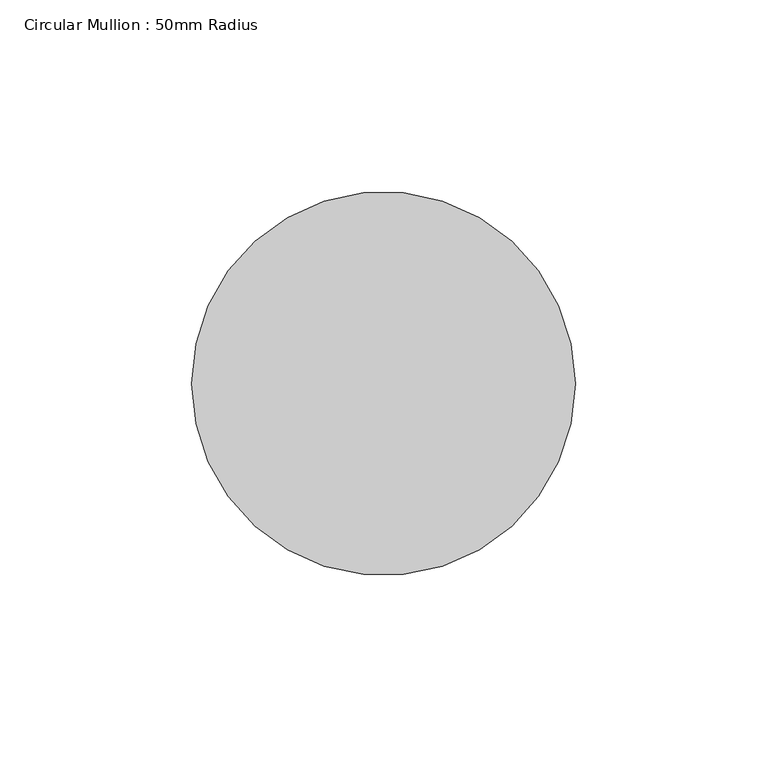
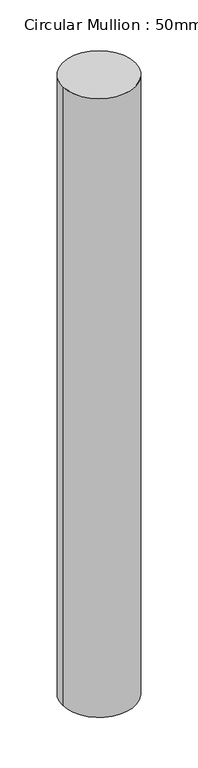
"""IFC4 building model written with IfcOpenShell, lengths in millimetres: member geometry, Circular Mullion : 50mm Radius."""

from ifc_helpers import new_model, si_unit, point, frame, origin, origin_2d, place, context, project, spatial, circle_curve, trimmed, segment, composite_curve, outline, extrude, source, transform, mapped, element, save


def circular_mullion_50mm_radius_d11fabc8(model_context):
    return source(origin(), model_context, "Body", "SweptSolid", [
        extrude(outline(composite_curve([segment(trimmed(circle_curve(origin_2d(), 50.0), [point((50.0, 0.0))], [point((-50.0, 0.0))], False, "CARTESIAN"), True, "CONTINUOUS"), segment(trimmed(circle_curve(origin_2d(), 50.0), [point((-50.0, 0.0))], [point((50.0, 0.0))], False, "CARTESIAN"), True, "CONTINUOUS")], self_intersect=False)), frame((0.0, 0.0, -903.1717388), z_axis=(0.0, 0.0, 1.0), x_axis=(1.0, 0.0, 0.0)), (0.0, 0.0, 1.0), 903.1717388),
    ])


if __name__ == "__main__":
    model = new_model("IFC4")
    model_context = context("Model", 3, world=origin())
    ifc_project = project(units=[si_unit("LENGTHUNIT", "METRE", prefix="MILLI")], contexts=[model_context])
    site = spatial("IfcSite", under=ifc_project)
    building = spatial("IfcBuilding", under=site)
    placement = place(None, origin())
    circular_mullion_50mm_radius_shape = circular_mullion_50mm_radius_d11fabc8(model_context)
    element("IfcMember", 1, ObjectType="Circular Mullion : 50mm Radius", at=placement, inside=building, context=model_context, shape_type="MappedRepresentation", body=[
        mapped(circular_mullion_50mm_radius_shape, transform((0.0, 0.0, 0.0), x_axis=(1.0, 0.0, 0.0), y_axis=(0.0, 1.0, 0.0), z_axis=(0.0, 0.0, 1.0))),
    ])
    save(model, "model.ifc")

# Revit data of these elements
# Type "Circular Mullion : 50mm Radius"
#   built-in parameter 1007350 = 0.164042 (stored number, unit not read)
# Element 1 (IfcMember, "Circular Mullion : 50mm Radius")
#   Materials on its faces: "Aluminium"
# Materials
#   "Aluminium": class "Metal", colour RGB 247 247 247, transparency 0, Description = "Aluminium 6061", Cost = 0
